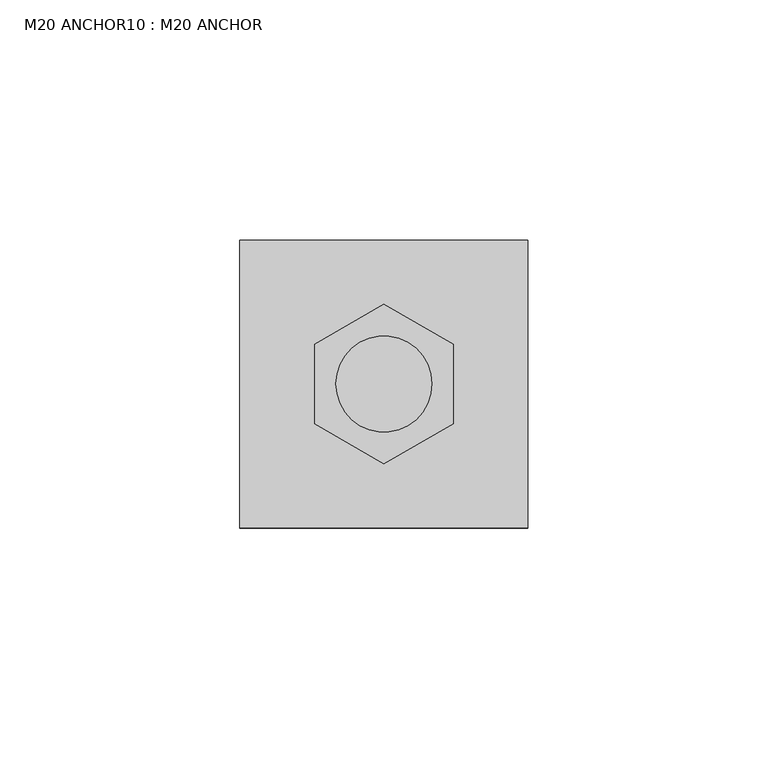
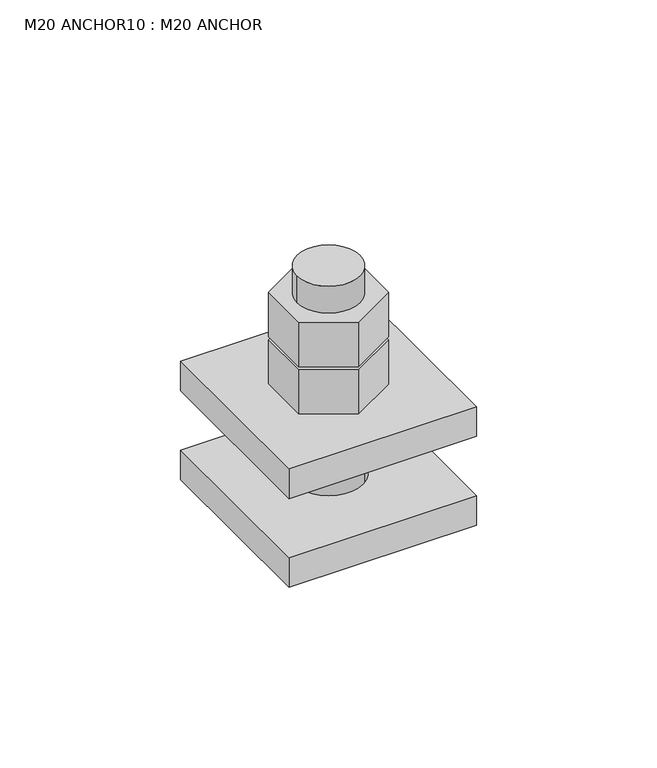
"""IFC4 building model written with IfcOpenShell, lengths in millimetres: fastener geometry, M20 ANCHOR10 : M20 ANCHOR."""

from ifc_helpers import new_model, si_unit, point, frame, frame_2d, origin, place, context, project, spatial, polyline, circle_curve, trimmed, segment, composite_curve, outline, extrude, source, transform, mapped, element, save


def m20_anchor10_m20_anchor_36d8eb8c(model_context):
    return source(origin(), model_context, "Body", "SweptSolid", [
        extrude(outline(polyline([(-8.0855968, 22453.9464399), (-22.4937158, 22445.6279085), (-36.9018348, 22453.9464399), (-36.9018348, 22470.5835027), (-22.4937158, 22478.9020341), (-8.0855968, 22470.5835027), (-8.0855968, 22453.9464399)]), holes=[composite_curve([segment(trimmed(circle_curve(frame_2d((-22.4937158, 22462.2649713)), 10.0), [point((-32.4937158, 22462.2649713))], [point((-12.4937158, 22462.2649713))], True, "CARTESIAN"), True, "CONTINUOUS"), segment(trimmed(circle_curve(frame_2d((-22.4937158, 22462.2649713)), 10.0), [point((-12.4937158, 22462.2649713))], [point((-32.4937158, 22462.2649713))], True, "CARTESIAN"), True, "CONTINUOUS")], self_intersect=False)]), frame((0.0, 0.0, 246.0), z_axis=(0.0, 0.0, 1.0), x_axis=(1.0, 0.0, 0.0)), (0.0, 0.0, 1.0), 15.0),
        extrude(outline(polyline([(-8.0855968, 22453.9464399), (-22.4937158, 22445.6279085), (-36.9018348, 22453.9464399), (-36.9018348, 22470.5835027), (-22.4937158, 22478.9020341), (-8.0855968, 22470.5835027), (-8.0855968, 22453.9464399)]), holes=[composite_curve([segment(trimmed(circle_curve(frame_2d((-22.4937158, 22462.2649713)), 10.0), [point((-32.4937158, 22462.2649713))], [point((-12.4937158, 22462.2649713))], True, "CARTESIAN"), True, "CONTINUOUS"), segment(trimmed(circle_curve(frame_2d((-22.4937158, 22462.2649713)), 10.0), [point((-12.4937158, 22462.2649713))], [point((-32.4937158, 22462.2649713))], True, "CARTESIAN"), True, "CONTINUOUS")], self_intersect=False)]), frame((0.0, 0.0, 230.0), z_axis=(0.0, 0.0, 1.0), x_axis=(1.0, 0.0, 0.0)), (0.0, 0.0, 1.0), 15.0),
        extrude(outline(composite_curve([segment(trimmed(circle_curve(frame_2d((-22.4937158, 22462.2649713)), 10.0), [point((-32.4937158, 22462.2649713))], [point((-12.4937158, 22462.2649713))], False, "CARTESIAN"), True, "CONTINUOUS"), segment(trimmed(circle_curve(frame_2d((-22.4937158, 22462.2649713)), 10.0), [point((-12.4937158, 22462.2649713))], [point((-32.4937158, 22462.2649713))], False, "CARTESIAN"), True, "CONTINUOUS")], self_intersect=False)), frame((0.0, 0.0, 190.0), z_axis=(0.0, 0.0, 1.0), x_axis=(1.0, 0.0, 0.0)), (0.0, 0.0, 1.0), 80.0),
        extrude(outline(polyline([(7.5062842, 22432.2649713), (-52.4937158, 22432.2649713), (-52.4937158, 22492.2649713), (7.5062842, 22492.2649713), (7.5062842, 22432.2649713)]), holes=[composite_curve([segment(trimmed(circle_curve(frame_2d((-22.4937158, 22462.2649713)), 11.0), [point((-33.4937158, 22462.2649713))], [point((-11.4937158, 22462.2649713))], True, "CARTESIAN"), True, "CONTINUOUS"), segment(trimmed(circle_curve(frame_2d((-22.4937158, 22462.2649713)), 11.0), [point((-11.4937158, 22462.2649713))], [point((-33.4937158, 22462.2649713))], True, "CARTESIAN"), True, "CONTINUOUS")], self_intersect=False)]), frame((0.0, 0.0, 190.0), z_axis=(0.0, 0.0, 1.0), x_axis=(1.0, 0.0, 0.0)), (0.0, 0.0, 1.0), 10.0),
        extrude(outline(polyline([(7.5062842, 22432.2649713), (-52.4937158, 22432.2649713), (-52.4937158, 22492.2649713), (7.5062842, 22492.2649713), (7.5062842, 22432.2649713)]), holes=[composite_curve([segment(trimmed(circle_curve(frame_2d((-22.4937158, 22462.2649713)), 11.0), [point((-33.4937158, 22462.2649713))], [point((-11.4937158, 22462.2649713))], True, "CARTESIAN"), True, "CONTINUOUS"), segment(trimmed(circle_curve(frame_2d((-22.4937158, 22462.2649713)), 11.0), [point((-11.4937158, 22462.2649713))], [point((-33.4937158, 22462.2649713))], True, "CARTESIAN"), True, "CONTINUOUS")], self_intersect=False)]), frame((0.0, 0.0, 220.0), z_axis=(0.0, 0.0, 1.0), x_axis=(1.0, 0.0, 0.0)), (0.0, 0.0, 1.0), 10.0),
    ])


if __name__ == "__main__":
    model = new_model("IFC4")
    model_context = context("Model", 3, world=origin())
    ifc_project = project(units=[si_unit("LENGTHUNIT", "METRE", prefix="MILLI")], contexts=[model_context])
    site = spatial("IfcSite", under=ifc_project)
    building = spatial("IfcBuilding", under=site)
    placement = place(None, origin())
    m20_anchor10_m20_anchor_shape = m20_anchor10_m20_anchor_36d8eb8c(model_context)
    element("IfcFastener", 1, ObjectType="M20 ANCHOR10 : M20 ANCHOR", at=placement, inside=building, context=model_context, shape_type="MappedRepresentation", body=[
        mapped(m20_anchor10_m20_anchor_shape, transform((0.0, 0.0, 0.0), x_axis=(1.0, 0.0, 0.0), y_axis=(0.0, 1.0, 0.0), z_axis=(0.0, 0.0, 1.0))),
    ])
    save(model, "model.ifc")
